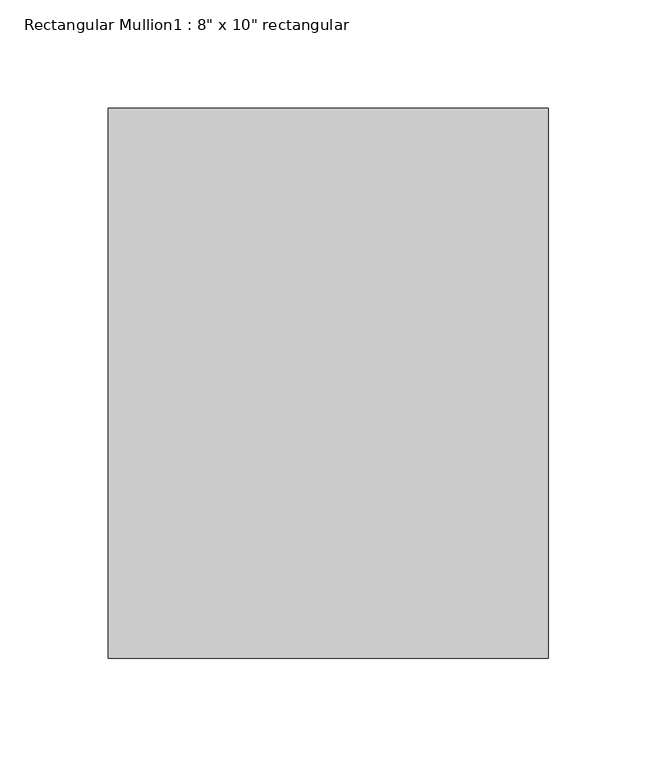
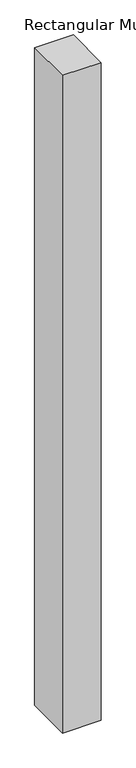
"""IFC4 building model written with IfcOpenShell, lengths in millimetres: member geometry."""

import ifcopenshell
import ifcopenshell.guid

model = None  # the IFC model being written
_history = None  # IfcOwnerHistory: only IFC2X3 demands one
_inside = {}  # id of a spatial element -> (the spatial element, [elements in it])
_under = {}  # id of a project, library or spatial element -> (it, [spatial elements below it])
_declared = {}  # id of a project -> (the project, [libraries it declares])
_typed = {}  # id of a type object -> (the type object, [elements of that type])
_made_of = {}  # id of a material, layer set ... -> (it, [elements and type objects made of it])


def new_model(schema):
    """Start an empty IFC model of exactly this schema.

    Asked for "IFC4X3", IfcOpenShell would pick the latest addendum, in which some entities
    have other attributes; the version numbers below select the first issue.
    IFC2X3 requires an IfcOwnerHistory on every rooted entity: one is made here for all.
    """
    global model, _history
    if schema == "IFC4X3":
        model = ifcopenshell.file(schema_version=(4, 3, 0, 0))
    else:
        model = ifcopenshell.file(schema=schema)
    _inside.clear()
    _under.clear()
    _declared.clear()
    _typed.clear()
    _made_of.clear()
    _history = None
    if model.schema == "IFC2X3":
        org = make("IfcOrganization", Name="unknown")
        user = make(
            "IfcPersonAndOrganization",
            ThePerson=make("IfcPerson", FamilyName="unknown"),
            TheOrganization=org,
        )
        app = make(
            "IfcApplication",
            ApplicationDeveloper=org,
            Version="unknown",
            ApplicationFullName="unknown",
            ApplicationIdentifier="unknown",
        )
        _history = make(
            "IfcOwnerHistory",
            OwningUser=user,
            OwningApplication=app,
            ChangeAction="ADDED",
            CreationDate=0,
        )
    return model


def make(cls, **values):
    """One entity of the class cls with the attributes given. An attribute that is None is left unset."""
    return model.create_entity(
        cls, **{name: value for name, value in values.items() if value is not None}
    )


def rooted(cls, **values):
    """An entity with a GlobalId (a new one), such as an element, a storey or a relation."""
    return make(cls, GlobalId=ifcopenshell.guid.new(), OwnerHistory=_history, **values)


def si_unit(unit_type, name, prefix=None):
    """IfcSIUnit, for example si_unit("LENGTHUNIT", "METRE", prefix="MILLI")."""
    return make("IfcSIUnit", UnitType=unit_type, Prefix=prefix, Name=name)


def assignment(units):
    """IfcUnitAssignment: the units of a project."""
    return None if units is None else make("IfcUnitAssignment", Units=units)


def point(xyz):
    """IfcCartesianPoint."""
    return None if xyz is None else make("IfcCartesianPoint", Coordinates=xyz)


def direction(xyz):
    """IfcDirection."""
    return None if xyz is None else make("IfcDirection", DirectionRatios=xyz)


def frame(location, z_axis=None, x_axis=None):
    """IfcAxis2Placement3D, a coordinate frame: its origin and axes. An axis left out is left unset."""
    return make(
        "IfcAxis2Placement3D",
        Location=point(location),
        Axis=direction(z_axis),
        RefDirection=direction(x_axis),
    )


def origin():
    """The frame at (0, 0, 0) with its axes left unset."""
    return frame((0.0, 0.0, 0.0))


def place(relative_to, where):
    """IfcLocalPlacement: puts the frame where relative to a parent placement (None: the world)."""
    return make(
        "IfcLocalPlacement", PlacementRelTo=relative_to, RelativePlacement=where
    )


def context(
    kind, dimensions, precision=None, world=None, true_north=None, identifier=None
):
    """IfcGeometricRepresentationContext, for example the 3D "Model" context."""
    return make(
        "IfcGeometricRepresentationContext",
        ContextIdentifier=identifier,
        ContextType=kind,
        CoordinateSpaceDimension=dimensions,
        Precision=precision,
        WorldCoordinateSystem=world,
        TrueNorth=true_north,
    )


def project(units=None, contexts=None):
    """IfcProject with its units and contexts."""
    return rooted(
        "IfcProject",
        Name="project",
        RepresentationContexts=contexts,
        UnitsInContext=assignment(units),
    )


def spatial(cls, under=None, at=None, **own):
    """A site, building, storey or space (cls), placed at a placement, below another one or the project."""
    s = rooted(cls, ObjectPlacement=at, **own)
    if under is not None:
        _under.setdefault(under.id(), (under, []))[1].append(s)
    return s


def polyline(points):
    """IfcPolyline through the points."""
    return make("IfcPolyline", Points=[point(p) for p in points])


def outline(outer, holes=None, kind="AREA"):
    """IfcArbitraryClosedProfileDef: a profile drawn as a closed curve; with holes, ...WithVoids."""
    if holes is None:
        return make("IfcArbitraryClosedProfileDef", ProfileType=kind, OuterCurve=outer)
    return make(
        "IfcArbitraryProfileDefWithVoids",
        ProfileType=kind,
        OuterCurve=outer,
        InnerCurves=holes,
    )


def extrude(swept, where, along, depth):
    """IfcExtrudedAreaSolid: the profile swept, set in the frame where, extruded along a direction by depth."""
    return make(
        "IfcExtrudedAreaSolid",
        SweptArea=swept,
        Position=where,
        ExtrudedDirection=direction(along),
        Depth=depth,
    )


def shape(context_of_items, identifier, shape_type, items):
    """IfcShapeRepresentation: the items that make up one representation, for example the "Body"."""
    return make(
        "IfcShapeRepresentation",
        ContextOfItems=context_of_items,
        RepresentationIdentifier=identifier,
        RepresentationType=shape_type,
        Items=items,
    )


def source(mapping_origin, context_of_items, identifier, shape_type, items):
    """IfcRepresentationMap: a shape defined once, which mapped items show again and again."""
    return make(
        "IfcRepresentationMap",
        MappingOrigin=mapping_origin,
        MappedRepresentation=shape(context_of_items, identifier, shape_type, items),
    )


def transform(
    local_origin,
    x_axis=None,
    y_axis=None,
    z_axis=None,
    scale=None,
    scale2=None,
    scale3=None,
    uniform=True,
):
    """IfcCartesianTransformationOperator3D, or its non-uniform kind. x_axis, y_axis, z_axis: its Axis1, 2, 3."""
    if uniform:
        return make(
            "IfcCartesianTransformationOperator3D",
            Axis1=direction(x_axis),
            Axis2=direction(y_axis),
            LocalOrigin=point(local_origin),
            Scale=scale,
            Axis3=direction(z_axis),
        )
    return make(
        "IfcCartesianTransformationOperator3DnonUniform",
        Axis1=direction(x_axis),
        Axis2=direction(y_axis),
        LocalOrigin=point(local_origin),
        Scale=scale,
        Axis3=direction(z_axis),
        Scale2=scale2,
        Scale3=scale3,
    )


def mapped(mapping_source, mapping_target):
    """IfcMappedItem: shows the shape of a source again, moved by a transform."""
    return make(
        "IfcMappedItem", MappingSource=mapping_source, MappingTarget=mapping_target
    )


def made_of(thing, what):
    """Note that an element or type object is made of a material, layer set ...; save() writes the relation."""
    if what is not None:
        _made_of.setdefault(what.id(), (what, []))[1].append(thing)
    return thing


def element(
    cls,
    number,
    at=None,
    inside=None,
    cuts=None,
    type_object=None,
    material=None,
    context=None,
    identifier="Body",
    shape_type=None,
    held_by="IfcProductDefinitionShape",
    body=None,
    shapes=None,
    **own,
):
    """One element of the class cls, such as IfcWall. Its Tag is "e" and its number.

    at: its placement. inside: the storey or other place that contains it. cuts: it is an
    opening in that element (IfcRelVoidsElement). A single representation is given by context,
    identifier, shape_type and body (its items); several are given by shapes. held_by: the class
    of the entity that holds the representations. save() writes the other relations.
    """
    e = rooted(cls, Tag="e%d" % number, ObjectPlacement=at, **own)
    if body is not None:
        shapes = [shape(context, identifier, shape_type, body)]
    if shapes is not None:
        e.Representation = make(held_by, Representations=shapes)
    if inside is not None:
        _inside.setdefault(inside.id(), (inside, []))[1].append(e)
    if cuts is not None:
        rooted(
            "IfcRelVoidsElement", RelatingBuildingElement=cuts, RelatedOpeningElement=e
        )
    if type_object is not None:
        _typed.setdefault(type_object.id(), (type_object, []))[1].append(e)
    return made_of(e, material)


def aggregate(whole, parts):
    """IfcRelAggregates: a whole, such as a stair, and the parts it consists of."""
    return rooted("IfcRelAggregates", RelatingObject=whole, RelatedObjects=parts)


def save(model, path):
    """Write the relations noted so far, then the file.

    IfcRelAggregates (storeys below a building ...), IfcRelContainedInSpatialStructure (elements
    in a storey), IfcRelDefinesByType, IfcRelAssociatesMaterial and IfcRelDeclares: one each for
    every whole, place, type object, material and project.
    """
    for whole, parts in _under.values():
        aggregate(whole, parts)
    for where, things in _inside.values():
        rooted(
            "IfcRelContainedInSpatialStructure",
            RelatedElements=things,
            RelatingStructure=where,
        )
    for kind, things in _typed.values():
        rooted("IfcRelDefinesByType", RelatedObjects=things, RelatingType=kind)
    for what, things in _made_of.values():
        rooted("IfcRelAssociatesMaterial", RelatedObjects=things, RelatingMaterial=what)
    for by, libraries in _declared.values():
        rooted("IfcRelDeclares", RelatingContext=by, RelatedDefinitions=libraries)
    model.write(path)


def member_98c0bc9c(model_context):
    return source(origin(), model_context, "Body", "SweptSolid", [
        extrude(outline(polyline([(0.0, 127.0), (0.0, -127.0), (-203.2, -127.0), (-203.2, 127.0), (0.0, 127.0)])), frame((0.0, 0.0, -3657.6), z_axis=(0.0, 0.0, 1.0), x_axis=(1.0, 0.0, 0.0)), (0.0, 0.0, 1.0), 3657.6),
    ])


if __name__ == "__main__":
    model = new_model("IFC4")
    model_context = context("Model", 3, world=origin())
    ifc_project = project(units=[si_unit("LENGTHUNIT", "METRE", prefix="MILLI")], contexts=[model_context])
    site = spatial("IfcSite", under=ifc_project)
    building = spatial("IfcBuilding", under=site)
    placement = place(None, origin())
    member_shape = member_98c0bc9c(model_context)
    element("IfcMember", 1, ObjectType="Rectangular Mullion1 : 8\" x 10\" rectangular", at=placement, inside=building, context=model_context, shape_type="MappedRepresentation", body=[
        mapped(member_shape, transform((0.0, 0.0, 0.0), x_axis=(1.0, 0.0, 0.0), y_axis=(0.0, 1.0, 0.0), z_axis=(0.0, 0.0, 1.0))),
    ])
    save(model, "model.ifc")

# Revit data of these elements
# Type "Rectangular Mullion1 : 8\" x 10\" rectangular"
#   built-in parameter 1007304 = 0.833333 (stored number, unit not read)
#   built-in parameter 1007301 = 0.333333 (stored number, unit not read)
#   built-in parameter 1007300 = 0.333333 (stored number, unit not read)
# Element 1 (IfcMember, "Rectangular Mullion1 : 8\" x 10\" rectangular")
#   Materials on its faces: "support-frame"
# Materials
#   "support-frame": class "Unassigned", colour RGB 233 233 233, transparency 0, Cost = 0
